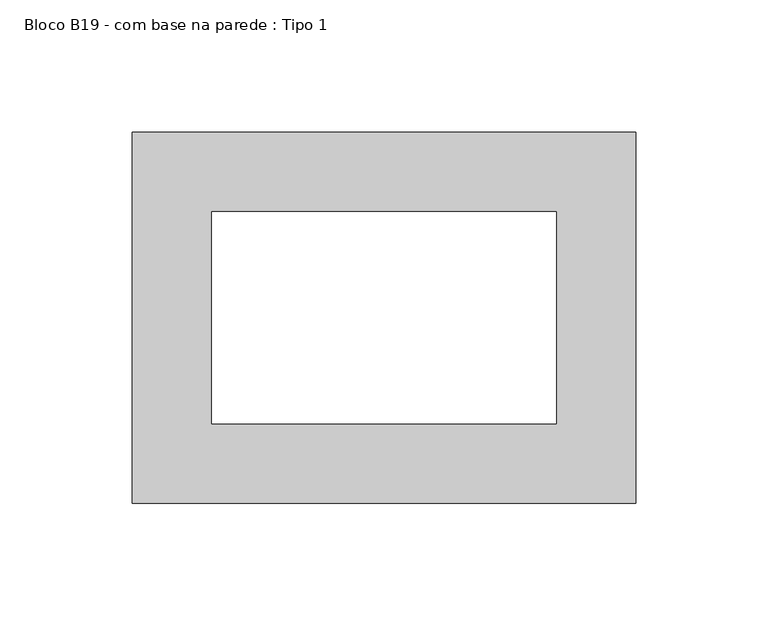
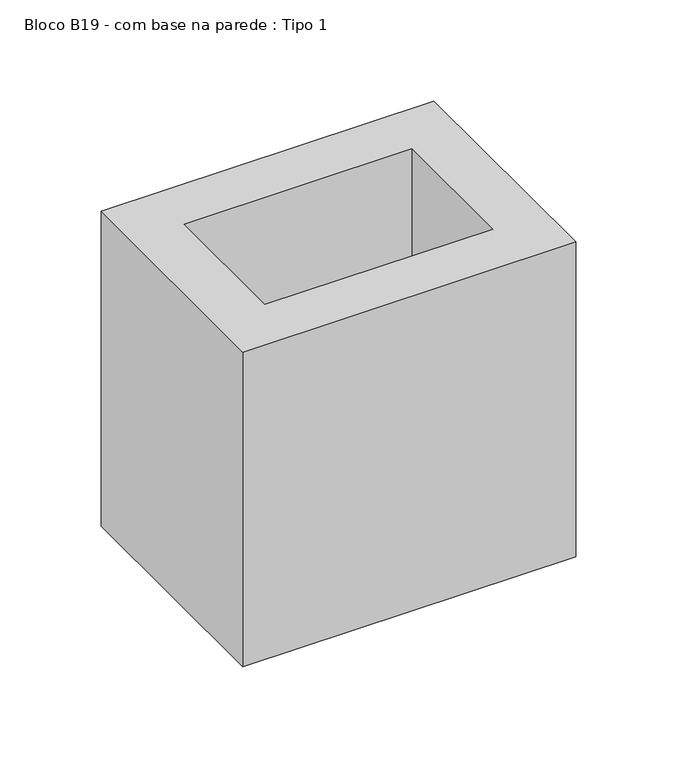
"""IFC4 building model written with IfcOpenShell, lengths in millimetres: proxy geometry, Bloco B19 - com base na parede : Tipo 1."""

from ifc_helpers import new_model, si_unit, origin, origin_with_axes, place, context, project, spatial, polyline, outline, extrude, source, transform, mapped, element, save


def bloco_b19_com_base_na_parede_tipo_1_d826db84(model_context):
    return source(origin(), model_context, "Body", "SweptSolid", [
        extrude(outline(polyline([(220.0, 70.0), (220.0, -70.0), (30.0, -70.0), (30.0, 70.0), (220.0, 70.0)]), holes=[polyline([(60.0, 40.0), (60.0, -40.0), (190.0, -40.0), (190.0, 40.0), (60.0, 40.0)])]), origin_with_axes(), (0.0, 0.0, 1.0), 190.0),
    ])


if __name__ == "__main__":
    model = new_model("IFC4")
    model_context = context("Model", 3, world=origin())
    ifc_project = project(units=[si_unit("LENGTHUNIT", "METRE", prefix="MILLI")], contexts=[model_context])
    site = spatial("IfcSite", under=ifc_project)
    building = spatial("IfcBuilding", under=site)
    placement = place(None, origin())
    bloco_b19_com_base_na_parede_tipo_1_shape = bloco_b19_com_base_na_parede_tipo_1_d826db84(model_context)
    element("IfcBuildingElementProxy", 1, Name="Bloco B19 - com base na parede : Tipo 1", ObjectType="Bloco B19 - com base na parede : Tipo 1", at=placement, inside=building, context=model_context, shape_type="MappedRepresentation", body=[
        mapped(bloco_b19_com_base_na_parede_tipo_1_shape, transform((0.0, 0.0, 0.0), x_axis=(1.0, 0.0, 0.0), y_axis=(0.0, 1.0, 0.0), z_axis=(0.0, 0.0, 1.0))),
    ])
    save(model, "model.ifc")

# Revit data of these elements
# Type "Bloco B19 - com base na parede : Tipo 1"
#   SINAPI = ""
#   Assembly Code = ""
